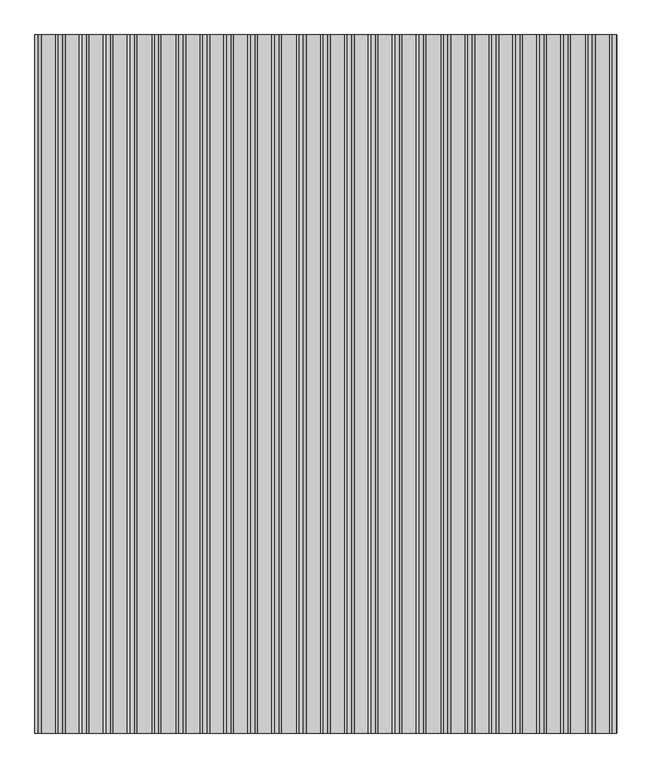
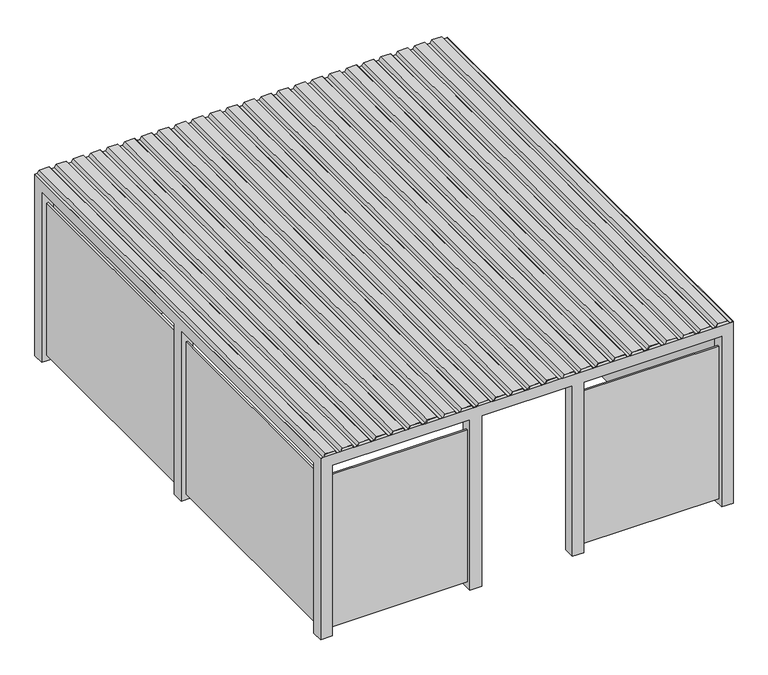
"""IFC4 building model written with IfcOpenShell, lengths in millimetres: proxy geometry, NLRS_90_GM_WPB_fietsenstalling-dicht_gen_rsf : fietsenstalling bxd 5000x6000mm."""

from ifc_helpers import new_model, si_unit, frame, origin, place, context, project, spatial, polyline, outline, extrude, faceted_brep, source, transform, mapped, element, save


def generic_models_cd129c34(model_context):
    return source(origin(), model_context, "Body", "SolidModel", [
        extrude(outline(polyline([(2361.0, -2446.0022315), (2361.0, -2326.9992824), (2326.0, -2303.0007176), (2326.0, -2263.0007963), (2361.0, -2239.0022315), (2361.0, -2119.9992824), (2326.0, -2096.0007176), (2326.0, -2056.0007963), (2361.0, -2032.0022315), (2361.0, -1912.9992824), (2326.0, -1889.0007176), (2326.0, -1849.0007963), (2361.0, -1825.0022315), (2361.0, -1705.9992824), (2326.0, -1682.0007176), (2326.0, -1642.0007963), (2361.0, -1618.0022315), (2361.0, -1498.9992824), (2326.0, -1475.0007176), (2326.0, -1434.9987283), (2361.0, -1411.0001636), (2361.0, -1291.9972144), (2326.0, -1267.9986497), (2326.0, -1227.9987283), (2361.0, -1204.0001636), (2361.0, -1084.9972144), (2326.0, -1060.9986497), (2326.0, -1020.9987283), (2361.0, -997.0001636), (2361.0, -877.9972144), (2326.0, -853.9986497), (2326.0, -813.9987283), (2361.0, -790.0001636), (2361.0, -670.9972144), (2326.0, -646.9986497), (2326.0, -606.9987283), (2361.0, -583.0001636), (2361.0, -463.9972144), (2326.0, -439.9986497), (2326.0, -399.9966604), (2361.0, -375.9980957), (2361.0, -256.9951465), (2326.0, -232.9965818), (2326.0, -192.9966604), (2361.0, -168.9980957), (2361.0, -49.9951465), (2326.0, -25.9965818), (2326.0, 14.0033396), (2361.0, 38.0019043), (2361.0, 157.0048535), (2326.0, 181.0034182), (2326.0, 221.0033396), (2361.0, 245.0019043), (2361.0, 364.0048535), (2326.0, 388.0034182), (2326.0, 428.0033396), (2361.0, 452.0019043), (2361.0, 571.0048535), (2326.0, 595.0034182), (2326.0, 635.0054075), (2361.0, 659.0039722), (2361.0, 778.0069214), (2326.0, 802.0054861), (2326.0, 842.0054075), (2361.0, 866.0039722), (2361.0, 985.0069214), (2326.0, 1009.0054861), (2326.0, 1049.0054075), (2361.0, 1073.0039722), (2361.0, 1192.0069214), (2326.0, 1216.0054861), (2326.0, 1256.0054075), (2361.0, 1280.0039722), (2361.0, 1399.0069214), (2326.0, 1423.0054861), (2326.0, 1463.0054075), (2361.0, 1487.0039722), (2361.0, 1606.0069214), (2326.0, 1630.0054861), (2326.0, 1670.0074754), (2361.0, 1694.0060401), (2361.0, 1813.0089893), (2326.0, 1837.007554), (2326.0, 1877.0074754), (2361.0, 1901.0060401), (2361.0, 2020.0089893), (2326.0, 2044.007554), (2326.0, 2084.0074754), (2361.0, 2108.0060401), (2361.0, 2227.0089893), (2326.0, 2251.007554), (2326.0, 2291.0074754), (2361.0, 2315.0060401), (2361.0, 2434.0089893), (2326.0, 2458.007554), (2326.0, 2498.0074754), (2328.9059388, 2500.0), (2332.4425986, 2500.0), (2328.0, 2496.9538289), (2328.0, 2459.0612005), (2363.0, 2435.0626358), (2363.0, 2313.9523936), (2328.0, 2289.9538289), (2328.0, 2252.0612005), (2363.0, 2228.0626358), (2363.0, 2106.9523936), (2328.0, 2082.9538289), (2328.0, 2045.0612005), (2363.0, 2021.0626358), (2363.0, 1899.9523936), (2328.0, 1875.9538289), (2328.0, 1838.0612005), (2363.0, 1814.0626358), (2363.0, 1692.9523936), (2328.0, 1668.9538289), (2328.0, 1631.0591326), (2363.0, 1607.0605679), (2363.0, 1485.9503257), (2328.0, 1461.951761), (2328.0, 1424.0591326), (2363.0, 1400.0605679), (2363.0, 1278.9503257), (2328.0, 1254.951761), (2328.0, 1217.0591326), (2363.0, 1193.0605679), (2363.0, 1071.9503257), (2328.0, 1047.951761), (2328.0, 1010.0591326), (2363.0, 986.0605679), (2363.0, 864.9503257), (2328.0, 840.951761), (2328.0, 803.0591326), (2363.0, 779.0605679), (2363.0, 657.9503257), (2328.0, 633.951761), (2328.0, 596.0570647), (2363.0, 572.0585), (2363.0, 450.9482578), (2328.0, 426.9496931), (2328.0, 389.0570647), (2363.0, 365.0585), (2363.0, 243.9482578), (2328.0, 219.9496931), (2328.0, 182.0570647), (2363.0, 158.0585), (2363.0, 36.9482578), (2328.0, 12.9496931), (2328.0, -24.9429353), (2363.0, -48.9415), (2363.0, -170.0517422), (2328.0, -194.0503069), (2328.0, -231.9429353), (2363.0, -255.9415), (2363.0, -377.0517422), (2328.0, -401.0503069), (2328.0, -438.9450032), (2363.0, -462.9435679), (2363.0, -584.0538101), (2328.0, -608.0523749), (2328.0, -645.9450032), (2363.0, -669.9435679), (2363.0, -791.0538101), (2328.0, -815.0523749), (2328.0, -852.9450032), (2363.0, -876.9435679), (2363.0, -998.0538101), (2328.0, -1022.0523749), (2328.0, -1059.9450032), (2363.0, -1083.9435679), (2363.0, -1205.0538101), (2328.0, -1229.0523749), (2328.0, -1266.9450032), (2363.0, -1290.9435679), (2363.0, -1412.0538101), (2328.0, -1436.0523749), (2328.0, -1473.9470711), (2363.0, -1497.9456358), (2363.0, -1619.055878), (2328.0, -1643.0544428), (2328.0, -1680.9470711), (2363.0, -1704.9456358), (2363.0, -1826.055878), (2328.0, -1850.0544428), (2328.0, -1887.9470711), (2363.0, -1911.9456358), (2363.0, -2033.055878), (2328.0, -2057.0544428), (2328.0, -2094.9470711), (2363.0, -2118.9456358), (2363.0, -2240.055878), (2328.0, -2264.0544428), (2328.0, -2301.9470711), (2363.0, -2325.9456358), (2363.0, -2447.055878), (2328.0, -2471.0544428), (2328.0, -2500.0), (2326.0, -2500.0), (2326.0, -2470.0007963), (2361.0, -2446.0022315)])), frame((0.0, -3000.0, 0.0), z_axis=(0.0, 1.0, 0.0), x_axis=(0.0, 0.0, 1.0)), (0.0, 0.0, 1.0), 6000.0),
        faceted_brep([(-690.0, 2940.0, 2023.0), (-2360.0, 2940.0, 2023.0), (-2360.0, 2920.0, 2023.0), (-690.0, 2920.0, 2023.0), (550.0, 2940.0, 2023.0), (-550.0, 2940.0, 2023.0), (-550.0, 2920.0, 2023.0), (550.0, 2920.0, 2023.0), (2360.0, 2940.0, 2023.0), (690.0, 2940.0, 2023.0), (690.0, 2920.0, 2023.0), (2360.0, 2920.0, 2023.0), (-2440.0, 2860.0, 2023.0), (-2440.0, 70.0, 2023.0), (-2420.0, 70.0, 2023.0), (-2420.0, 2860.0, 2023.0), (-2440.0, -70.0, 2023.0), (-2440.0, -2860.0, 2023.0), (-2420.0, -2860.0, 2023.0), (-2420.0, -70.0, 2023.0), (-2360.0, -2940.0, 2023.0), (-690.0, -2940.0, 2023.0), (-690.0, -2920.0, 2023.0), (-2360.0, -2920.0, 2023.0), (2420.0, 2860.0, 2023.0), (2420.0, 70.0, 2023.0), (2440.0, 70.0, 2023.0), (2440.0, 2860.0, 2023.0), (2420.0, -70.0, 2023.0), (2420.0, -2860.0, 2023.0), (2440.0, -2860.0, 2023.0), (2440.0, -70.0, 2023.0), (2360.0, -2920.0, 2023.0), (690.0, -2920.0, 2023.0), (690.0, -2940.0, 2023.0), (2360.0, -2940.0, 2023.0), (2440.0, 2860.0, 70.0), (2440.0, 70.0, 70.0), (2420.0, 70.0, 70.0), (2420.0, 2860.0, 70.0), (2440.0, -70.0, 70.0), (2440.0, -2860.0, 70.0), (2420.0, -2860.0, 70.0), (2420.0, -70.0, 70.0), (2360.0, -2940.0, 70.0), (690.0, -2940.0, 70.0), (690.0, -2920.0, 70.0), (2360.0, -2920.0, 70.0), (-690.0, 2920.0, 70.0), (-2360.0, 2920.0, 70.0), (-2360.0, 2940.0, 70.0), (-690.0, 2940.0, 70.0), (550.0, 2920.0, 70.0), (-550.0, 2920.0, 70.0), (-550.0, 2940.0, 70.0), (550.0, 2940.0, 70.0), (2360.0, 2920.0, 70.0), (690.0, 2920.0, 70.0), (690.0, 2940.0, 70.0), (2360.0, 2940.0, 70.0), (-2420.0, 2860.0, 70.0), (-2420.0, 70.0, 70.0), (-2440.0, 70.0, 70.0), (-2440.0, 2860.0, 70.0), (-2420.0, -70.0, 70.0), (-2420.0, -2860.0, 70.0), (-2440.0, -2860.0, 70.0), (-2440.0, -70.0, 70.0), (-2360.0, -2920.0, 70.0), (-690.0, -2920.0, 70.0), (-690.0, -2940.0, 70.0), (-2360.0, -2940.0, 70.0), (-2360.0, 3000.0, 0.0), (-2360.0, 2860.0, 0.0), (-2500.0, 2860.0, 0.0), (-2500.0, 3000.0, 0.0), (-2360.0, -2860.0, 0.0), (-2360.0, -3000.0, 0.0), (-2500.0, -3000.0, 0.0), (-2500.0, -2860.0, 0.0), (2500.0, 3000.0, 0.0), (2500.0, 2860.0, 0.0), (2360.0, 2860.0, 0.0), (2360.0, 3000.0, 0.0), (2500.0, -2860.0, 0.0), (2500.0, -3000.0, 0.0), (2360.0, -3000.0, 0.0), (2360.0, -2860.0, 0.0), (-2360.0, 70.0, 0.0), (-2360.0, -70.0, 0.0), (-2500.0, -70.0, 0.0), (-2500.0, 70.0, 0.0), (2500.0, 70.0, 0.0), (2500.0, -70.0, 0.0), (2360.0, -70.0, 0.0), (2360.0, 70.0, 0.0), (-550.0, 3000.0, 0.0), (-550.0, 2860.0, 0.0), (-690.0, 2860.0, 0.0), (-690.0, 3000.0, 0.0), (690.0, 3000.0, 0.0), (690.0, 2860.0, 0.0), (550.0, 2860.0, 0.0), (550.0, 3000.0, 0.0), (-550.0, -2860.0, 0.0), (-550.0, -3000.0, 0.0), (-690.0, -3000.0, 0.0), (-690.0, -2860.0, 0.0), (690.0, -2860.0, 0.0), (690.0, -3000.0, 0.0), (550.0, -3000.0, 0.0), (550.0, -2860.0, 0.0), (-2500.0, 3000.0, 2326.0), (2500.0, 3000.0, 2326.0), (2360.0, 3000.0, 2186.0), (690.0, 3000.0, 2186.0), (550.0, 3000.0, 2186.0), (-550.0, 3000.0, 2186.0), (-690.0, 3000.0, 2186.0), (-2360.0, 3000.0, 2186.0), (-2500.0, 2860.0, 2186.0), (-2500.0, 70.0, 2186.0), (-2500.0, -70.0, 2186.0), (-2500.0, -2860.0, 2186.0), (-2500.0, -3000.0, 2326.0), (-2360.0, 2860.0, 2186.0), (-2360.0, -2860.0, 2186.0), (-2360.0, -3000.0, 2186.0), (-690.0, -3000.0, 2186.0), (-550.0, -3000.0, 2186.0), (550.0, -3000.0, 2186.0), (690.0, -3000.0, 2186.0), (2360.0, -3000.0, 2186.0), (2500.0, -3000.0, 2326.0), (2360.0, 2860.0, 2186.0), (2500.0, 2860.0, 2186.0), (2500.0, -2860.0, 2186.0), (2500.0, -70.0, 2186.0), (2500.0, 70.0, 2186.0), (2360.0, -2860.0, 2186.0), (-2360.0, 70.0, 2186.0), (-2360.0, -70.0, 2186.0), (-2360.0, 2860.0, 2326.0), (-2360.0, -2860.0, 2326.0), (2360.0, 70.0, 2186.0), (2360.0, -70.0, 2186.0), (2360.0, -2860.0, 2326.0), (2360.0, 2860.0, 2326.0), (-690.0, 2860.0, 2186.0), (-550.0, 2860.0, 2186.0), (550.0, 2860.0, 2186.0), (690.0, 2860.0, 2186.0), (-690.0, -2860.0, 2186.0), (690.0, -2860.0, 2186.0), (550.0, -2860.0, 2186.0), (-550.0, -2860.0, 2186.0)], [[[0, 1, 2, 3]], [[4, 5, 6, 7]], [[8, 9, 10, 11]], [[12, 13, 14, 15]], [[16, 17, 18, 19]], [[20, 21, 22, 23]], [[24, 25, 26, 27]], [[28, 29, 30, 31]], [[32, 33, 34, 35]], [[36, 37, 38, 39]], [[40, 41, 42, 43]], [[44, 45, 46, 47]], [[48, 49, 50, 51]], [[52, 53, 54, 55]], [[56, 57, 58, 59]], [[60, 61, 62, 63]], [[64, 65, 66, 67]], [[68, 69, 70, 71]], [[1, 0, 51, 50]], [[5, 4, 55, 54]], [[9, 8, 59, 58]], [[13, 12, 63, 62]], [[17, 16, 67, 66]], [[21, 20, 71, 70]], [[23, 22, 69, 68]], [[15, 14, 61, 60]], [[19, 18, 65, 64]], [[3, 2, 49, 48]], [[7, 6, 53, 52]], [[11, 10, 57, 56]], [[25, 24, 39, 38]], [[29, 28, 43, 42]], [[33, 32, 47, 46]], [[35, 34, 45, 44]], [[27, 26, 37, 36]], [[31, 30, 41, 40]], [[72, 73, 74, 75]], [[76, 77, 78, 79]], [[80, 81, 82, 83]], [[84, 85, 86, 87]], [[88, 89, 90, 91]], [[92, 93, 94, 95]], [[96, 97, 98, 99]], [[100, 101, 102, 103]], [[104, 105, 106, 107]], [[108, 109, 110, 111]], [[72, 75, 112, 113, 80, 83, 114, 115, 100, 103, 116, 117, 96, 99, 118, 119]], [[112, 75, 74, 120, 121, 91, 90, 122, 123, 79, 78, 124]], [[74, 73, 125, 120], [12, 15, 60, 63]], [[73, 72, 119, 125], [2, 1, 50, 49]], [[76, 79, 123, 126], [18, 17, 66, 65]], [[124, 78, 77, 127, 128, 106, 105, 129, 130, 110, 109, 131, 132, 86, 85, 133]], [[77, 76, 126, 127], [20, 23, 68, 71]], [[83, 82, 134, 114], [8, 11, 56, 59]], [[82, 81, 135, 134], [24, 27, 36, 39]], [[81, 80, 113, 133, 85, 84, 136, 137, 93, 92, 138, 135]], [[84, 87, 139, 136], [30, 29, 42, 41]], [[87, 86, 132, 139], [32, 35, 44, 47]], [[88, 91, 121, 140], [14, 13, 62, 61]], [[90, 89, 141, 122], [16, 19, 64, 67]], [[89, 88, 140, 125, 142, 143, 126, 141]], [[92, 95, 144, 138], [26, 25, 38, 37]], [[95, 94, 145, 139, 146, 147, 134, 144]], [[94, 93, 137, 145], [28, 31, 40, 43]], [[99, 98, 148, 118], [0, 3, 48, 51]], [[98, 97, 149, 150, 102, 101, 151, 134, 147, 142, 125, 148]], [[97, 96, 117, 149], [6, 5, 54, 53]], [[103, 102, 150, 116], [4, 7, 52, 55]], [[101, 100, 115, 151], [10, 9, 58, 57]], [[104, 107, 152, 126, 143, 146, 139, 153, 108, 111, 154, 155]], [[107, 106, 128, 152], [22, 21, 70, 69]], [[105, 104, 155, 129]], [[111, 110, 130, 154]], [[109, 108, 153, 131], [34, 33, 46, 45]], [[113, 112, 124, 133], [147, 146, 143, 142]], [[115, 114, 134, 151]], [[117, 116, 150, 149]], [[119, 118, 148, 125]], [[123, 122, 141, 126]], [[135, 138, 144, 134]], [[125, 140, 121, 120]], [[139, 145, 137, 136]], [[126, 152, 128, 127]], [[153, 139, 132, 131]], [[155, 154, 130, 129]]]),
    ])


if __name__ == "__main__":
    model = new_model("IFC4")
    model_context = context("Model", 3, world=origin())
    ifc_project = project(units=[si_unit("LENGTHUNIT", "METRE", prefix="MILLI")], contexts=[model_context])
    site = spatial("IfcSite", under=ifc_project)
    building = spatial("IfcBuilding", under=site)
    placement = place(None, origin())
    generic_models_shape = generic_models_cd129c34(model_context)
    element("IfcBuildingElementProxy", 1, Name="NLRS_90_GM_WPB_fietsenstalling-dicht_gen_rsf : fietsenstalling bxd 5000x6000mm", ObjectType="NLRS_90_GM_WPB_fietsenstalling-dicht_gen_rsf : fietsenstalling bxd 5000x6000mm", at=placement, inside=building, context=model_context, shape_type="MappedRepresentation", body=[
        mapped(generic_models_shape, transform((0.0, 0.0, 0.0), x_axis=(1.0, 0.0, 0.0), y_axis=(0.0, 1.0, 0.0), z_axis=(0.0, 0.0, 1.0))),
    ])
    save(model, "model.ifc")

# Revit data of these elements
# Type "NLRS_90_GM_WPB_fietsenstalling-dicht_gen_rsf : fietsenstalling bxd 5000x6000mm"
#   Type IFC Predefined Type = "USERDEFINED"
#   Export Type to IFC As = "IfcGeographicElementType"
#   Type IfcGUID = "05J6pyYiTDtR2exmlhyQiW"
#   Description = "fietsenstalling open bxdxh 5000x2000x2300mm"
#   IfcName[Type] = "fietsenstalling bxd 5000x6000mm"
#   IfcDescription[Type] = "fietsenstalling open bxdxh 5000x2000x2300mm"
#   IfcObjectType[Type] = "BICYCLE_STORAGE"
#   IfcExportAs[Type] = "IfcGeographicElementType"
#   IfcExportType[Type] = "USERDEFINED"
#   NLRS_C_omschrijving_02 [instance default] = "wanden"
#   NLRS_C_omschrijving_01 [instance default] = "dak"
#   NLRS_C_omschrijving [instance default] = "constructie"
#   NLRS_C_materiaal_afwerking_02 [instance default] = ""
#   NLRS_C_materiaal_afwerking_01 [instance default] = ""
#   NLRS_C_materiaal_afwerking [instance default] = ""
#   Model = "generiek"
#   Manufacturer = "generiek"
#   Assembly Code = "90.22"
#   wand_dikte = 20.00 mm
#   constructie_dikte = 140.00 mm
#   NLRS_S_gewicht [instance default] = 0.00 kg
#   NLRS_C_oppervlakte = 30.00 m²
#   NLRS_C_hoogte = 2326.00 mm
#   NLRS_C_diepte = 6000.00 mm
#   NLRS_C_breedte = 5000.00 mm
#   Default Elevation = 1219.20 mm
#   NLRS_C_buiten [instance default] = yes
#   NLRS_C_materiaal_02 = none
#   NLRS_C_materiaal_01 = none
#   NLRS_C_materiaal = none
#   URL = ""
